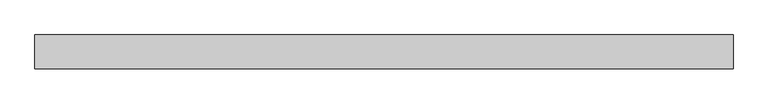
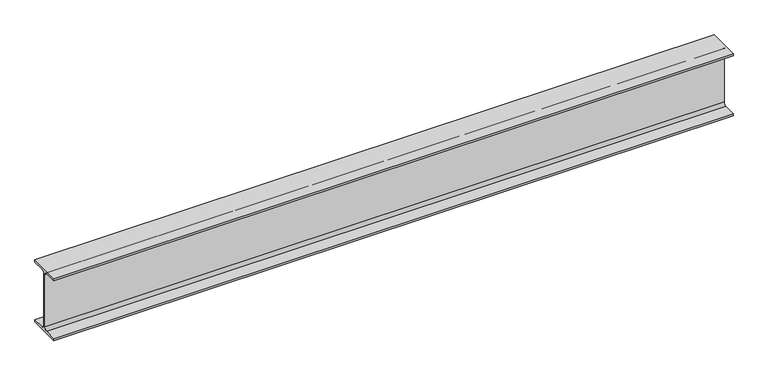
"""IFC4 building model written with IfcOpenShell, lengths in millimetres: beam geometry, 0912_Steel Framing_H-KSD3502 : H_SB_ASB_H-250x125x6x9."""

from ifc_helpers import new_model, si_unit, point, frame, frame_2d, origin, place, context, project, spatial, polyline, circle_curve, trimmed, segment, composite_curve, outline, extrude, source, transform, mapped, element, save


def beam_97715b9d(model_context):
    return source(origin(), model_context, "Body", "SweptSolid", [
        extrude(outline(composite_curve([segment(polyline([(62.5, -116.0), (62.5, -125.0), (-62.5, -125.0), (-62.5, -116.0), (-15.0, -116.0)]), True, "CONTINUOUS"), segment(trimmed(circle_curve(frame_2d((-15.0, -104.0)), 12.0), [point((-15.0, -116.0))], [point((-3.0, -104.0))], True, "CARTESIAN"), True, "CONTINUOUS"), segment(polyline([(-3.0, -104.0), (-3.0, 104.0)]), True, "CONTINUOUS"), segment(trimmed(circle_curve(frame_2d((-15.0, 104.0)), 12.0), [point((-3.0, 104.0))], [point((-15.0, 116.0))], True, "CARTESIAN"), True, "CONTINUOUS"), segment(polyline([(-15.0, 116.0), (-62.5, 116.0), (-62.5, 125.0), (62.5, 125.0), (62.5, 116.0), (15.0, 116.0)]), True, "CONTINUOUS"), segment(trimmed(circle_curve(frame_2d((15.0, 104.0)), 12.0), [point((15.0, 116.0))], [point((3.0, 104.0))], True, "CARTESIAN"), True, "CONTINUOUS"), segment(polyline([(3.0, 104.0), (3.0, -104.0)]), True, "CONTINUOUS"), segment(trimmed(circle_curve(frame_2d((15.0, -104.0)), 12.0), [point((3.0, -104.0))], [point((15.0, -116.0))], True, "CARTESIAN"), True, "CONTINUOUS"), segment(polyline([(15.0, -116.0), (62.5, -116.0)]), True, "CONTINUOUS")], self_intersect=False)), frame((-1249.3, 0.0, 0.0), z_axis=(1.0, 0.0, 0.0), x_axis=(0.0, 1.0, 0.0)), (0.0, 0.0, 1.0), 2586.6),
    ])


if __name__ == "__main__":
    model = new_model("IFC4")
    model_context = context("Model", 3, world=origin())
    ifc_project = project(units=[si_unit("LENGTHUNIT", "METRE", prefix="MILLI")], contexts=[model_context])
    site = spatial("IfcSite", under=ifc_project)
    building = spatial("IfcBuilding", under=site)
    placement = place(None, origin())
    beam_shape = beam_97715b9d(model_context)
    element("IfcBeam", 1, ObjectType="0912_Steel Framing_H-KSD3502 : H_SB_ASB_H-250x125x6x9", at=placement, inside=building, context=model_context, shape_type="MappedRepresentation", body=[
        mapped(beam_shape, transform((0.0, 0.0, 0.0), x_axis=(1.0, 0.0, 0.0), y_axis=(0.0, 1.0, 0.0), z_axis=(0.0, 0.0, 1.0))),
    ])
    save(model, "model.ifc")

# Revit data of these elements
# Type "0912_Steel Framing_H-KSD3502 : H_SB_ASB_H-250x125x6x9"
#   H_WM Code_1 = "S01AA003-00001 | Main Steel Structure Fabrication Work | Shelter/Building | Light Steel - Standard (30KG/M>Weight) | Material: (   )"
#   H_WM Code_2 = "S03AA029-00001 | Main Steel Structure Erection Work | Shelter/Building | Light Steel (30KG/M>Weight) | Material: (   )"
#   H_WM Code_3 = "S01AA010-00001 | Main Steel Structure Fabrication Work | Shelter/Building | Steel Painting/Coating | for Non-Fireproofed Steel Surface, Surface Preparation, Primer, Second & Final Coat | Material: (   )"
#   H_Q'ty Cal Type Tag = "SB-Q2"
#   Width = 12.5 cm
#   Web Thickness = 0.6 cm
#   Web Fillet = 1.2 cm
#   Warping Constant = 42539.8 cm⁶
#   W = 0
#   Torsional Moment of Inertia = 7.8102 cm⁴
#   Section Area = 37.66 cm²
#   Plastic Modulus weak axis = 73.1 cm³
#   Plastic Modulus strong axis = 366.0 cm³
#   Perimeter = 0.97 m²/m
#   Nominal Weight = 29.60 kgf/m
#   Moment of Inertia weak axis = 294.00 cm⁴
#   Moment of Inertia strong axis = 4050.00 cm⁴
#   Height = 25.0 cm
#   Flange Thickness = 0.9 cm
#   Elastic Modulus weak axis = 47.0 cm³
#   Elastic Modulus strong axis = 324.0 cm³
#   Centroid Vertical = 12.5 cm
#   Centroid Horizontal = 6.25 cm
#   Ix = 40500000
#   Length [instance default] = 1.5240 m
#   Zx = 366000
#   b = 0.1250 m
#   h = 0.2500 m
#   r = 0.0120 m
#   s = 0.0060 m
#   t = 0.0090 m
#   A = 0.003766 m²
#   Structural Material [instance default] = Steel, 45-345
#   Assembly Code = ""
# Element 1 (IfcBeam, "0912_Steel Framing_H-KSD3502 : H_SB_ASB_H-250x125x6x9")
#   Structural Material = none
# Materials
#   "Steel, 45-345": class "Metal", colour RGB 189 187 185, transparency 0, Description = "Steel 345 MPa", Cost = 0
